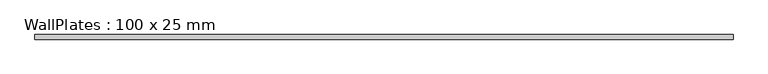
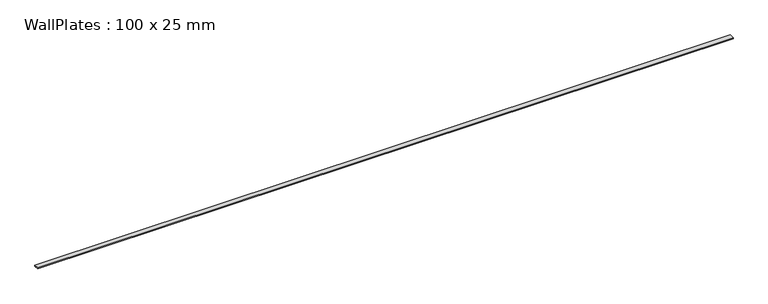
"""IFC4 building model written with IfcOpenShell, lengths in millimetres: beam geometry, WallPlates : 100 x 25 mm."""

from ifc_helpers import new_model, si_unit, frame, origin, place, context, project, spatial, polyline, outline, extrude, source, transform, mapped, element, save


def wallplates_100_x_25_mm_46d173e7(model_context):
    return source(origin(), model_context, "Body", "SweptSolid", [
        extrude(outline(polyline([(-7550.0, -50.0), (-7550.0, 50.0), (7550.0, 50.0), (7550.0, -50.0), (-7550.0, -50.0)])), frame((0.0, 0.0, -12.5), z_axis=(0.0, 0.0, 1.0), x_axis=(1.0, 0.0, 0.0)), (0.0, 0.0, 1.0), 25.0),
    ])


if __name__ == "__main__":
    model = new_model("IFC4")
    model_context = context("Model", 3, world=origin())
    ifc_project = project(units=[si_unit("LENGTHUNIT", "METRE", prefix="MILLI")], contexts=[model_context])
    site = spatial("IfcSite", under=ifc_project)
    building = spatial("IfcBuilding", under=site)
    placement = place(None, origin())
    wallplates_100_x_25_mm_shape = wallplates_100_x_25_mm_46d173e7(model_context)
    element("IfcBeam", 1, ObjectType="WallPlates : 100 x 25 mm", at=placement, inside=building, context=model_context, shape_type="MappedRepresentation", body=[
        mapped(wallplates_100_x_25_mm_shape, transform((0.0, 0.0, 0.0), x_axis=(1.0, 0.0, 0.0), y_axis=(0.0, 1.0, 0.0), z_axis=(0.0, 0.0, 1.0))),
    ])
    save(model, "model.ifc")

# Revit data of these elements
# Type "WallPlates : 100 x 25 mm"
#   ExpertTruss = "Height\th\r\nWidth\tb"
#   Name [instance default] = ""
#   m [instance default] = 0 mm
#   ip_c_cut [instance default] = 1025 mm
#   h_fix [instance default] = 75 mm
#   d/2 [instance default] = 1750 mm
#   c_cut_incl [instance default] = -1000 mm
#   c_cut [instance default] = 0 mm
#   alfaMax [instance default] = 0.00°
#   alfa0_2 [instance default] = 90.00°
#   Alfa_str [instance default] = 0.00°
#   Alfa_cut [instance default] = 90.00°
#   AlfaMAX [instance default] = 0.00°
#   Alfa2_0 [instance default] = 0.00°
#   Alfa2 [instance default] = 0.00°
#   Alfa1_0 [instance default] = 0.00°
#   Alfa1 [instance default] = 0.00°
#   A_max_Str [instance default] = 0.00°
#   h_void [instance default] = 25 mm
#   beam_L_0 [instance default] = 100 mm
#   beam_L [instance default] = 0 mm
#   b_void [instance default] = 110 mm
#   alfa0_1 [instance default] = 90.00°
#   b = 100 mm
#   YOffsetStr [instance default] = 0 mm
#   YOffsetEnd [instance default] = 0 mm
#   XOffsetStr_0 [instance default] = 3500 mm
#   XOffsetStr [instance default] = 0 mm
#   XOffsetEnd_0 [instance default] = 3500 mm
#   XOffsetEnd [instance default] = 0 mm
#   L_void_0 [instance default] = 100 mm
#   L_void [instance default] = 0 mm
#   E2 [instance default] = 0.00°
#   E1 [instance default] = 0.00°
#   Length [instance default] = 3500 mm
#   h = 25 mm
#   Alfa [instance default] = 0.00°
#   A_max_End [instance default] = 0.00°
#   A_max [instance default] = 0.00°
#   A4 [instance default] = 0.00°
#   A3 [instance default] = 0.00°
#   A2 [instance default] = 0.00°
#   A1 [instance default] = 0.00°
#   Material [instance default] = Wood Standard
# Element 1 (IfcBeam, "WallPlates : 100 x 25 mm")
#   d/2 = 7500 mm
#   XOffsetStr_0 = 15050 mm
#   XOffsetStr = -50 mm
#   XOffsetEnd_0 = 15050 mm
#   XOffsetEnd = -50 mm
#   Materials on its faces: "Wood Standard"
# Materials
#   "Wood Standard": class "Drewno", colour RGB 196 146 67, transparency 0, Cost = 0
